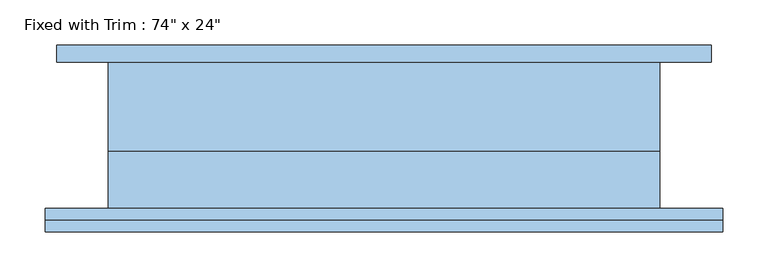
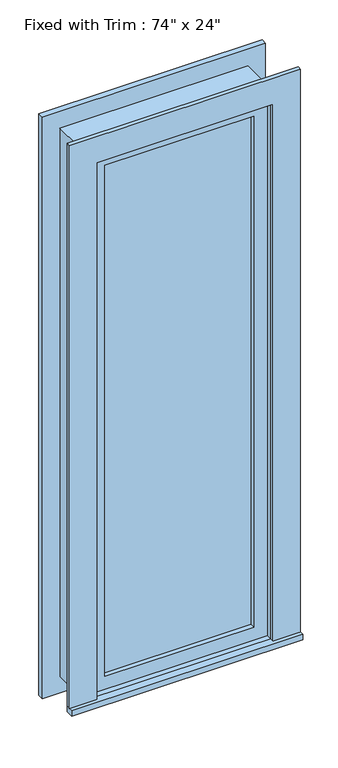
"""IFC4 building model written with IfcOpenShell, lengths in millimetres: window geometry."""

from ifc_helpers import new_model, si_unit, frame, origin, place, context, project, spatial, polyline, outline, extrude, source, transform, mapped, element, save


def window_368a6f6d(model_context):
    return source(origin(), model_context, "Body", "SweptSolid", [
        extrude(outline(polyline([(-412.75, -106.3625), (-412.75, -80.9625), (336.55, -80.9625), (336.55, -106.3625), (-412.75, -106.3625)])), frame((0.0, 0.0, 914.4), z_axis=(0.0, 0.0, 1.0), x_axis=(1.0, 0.0, 0.0)), (0.0, 0.0, 1.0), 19.05),
        extrude(outline(polyline([(2774.95, -323.85), (2774.95, 247.65), (933.45, 247.65), (933.45, 336.55), (2863.85, 336.55), (2863.85, -412.75), (933.45, -412.75), (933.45, -323.85), (2774.95, -323.85)])), frame((0.0, -93.6625, 0.0), z_axis=(0.0, 1.0, 0.0), x_axis=(0.0, 0.0, 1.0)), (0.0, 0.0, 1.0), 12.7),
        extrude(outline(polyline([(2851.15, 323.85), (2851.15, -400.05), (857.25, -400.05), (857.25, 323.85), (2851.15, 323.85)]), holes=[polyline([(2762.25, 234.95), (946.15, 234.95), (946.15, -311.15), (2762.25, -311.15), (2762.25, 234.95)])]), frame((0.0, 80.9625, 0.0), z_axis=(0.0, 1.0, 0.0), x_axis=(0.0, 0.0, 1.0)), (0.0, 0.0, 1.0), 19.05),
        extrude(outline(polyline([(203.2, -33.3375), (203.2, -46.0375), (-279.4, -46.0375), (-279.4, -33.3375), (203.2, -33.3375)])), frame((0.0, 0.0, 977.9), z_axis=(0.0, 0.0, 1.0), x_axis=(1.0, 0.0, 0.0)), (0.0, 0.0, 1.0), 1752.6),
        extrude(outline(polyline([(2774.95, -323.85), (933.45, -323.85), (933.45, 247.65), (2774.95, 247.65), (2774.95, -323.85)]), holes=[polyline([(2730.5, -279.4), (2730.5, 203.2), (977.9, 203.2), (977.9, -279.4), (2730.5, -279.4)])]), frame((0.0, -61.9125, 0.0), z_axis=(0.0, 1.0, 0.0), x_axis=(0.0, 0.0, 1.0)), (0.0, 0.0, 1.0), 44.45),
        extrude(outline(polyline([(2794.0, -342.9), (914.4, -342.9), (914.4, 266.7), (2794.0, 266.7), (2794.0, -342.9)]), holes=[polyline([(2762.25, -311.15), (2762.25, 234.95), (946.15, 234.95), (946.15, -311.15), (2762.25, -311.15)])]), frame((0.0, -17.4625, 0.0), z_axis=(0.0, 1.0, 0.0), x_axis=(0.0, 0.0, 1.0)), (0.0, 0.0, 1.0), 98.425),
        extrude(outline(polyline([(2794.0, 266.7), (2794.0, -342.9), (914.4, -342.9), (914.4, 266.7), (2794.0, 266.7)]), holes=[polyline([(2774.95, 247.65), (933.45, 247.65), (933.45, -323.85), (2774.95, -323.85), (2774.95, 247.65)])]), frame((0.0, -80.9625, 0.0), z_axis=(0.0, 1.0, 0.0), x_axis=(0.0, 0.0, 1.0)), (0.0, 0.0, 1.0), 63.5),
    ])


if __name__ == "__main__":
    model = new_model("IFC4")
    model_context = context("Model", 3, world=origin())
    ifc_project = project(units=[si_unit("LENGTHUNIT", "METRE", prefix="MILLI")], contexts=[model_context])
    site = spatial("IfcSite", under=ifc_project)
    building = spatial("IfcBuilding", under=site)
    placement = place(None, origin())
    window_shape = window_368a6f6d(model_context)
    element("IfcWindow", 1, ObjectType="Fixed with Trim : 74\" x 24\"", at=placement, inside=building, context=model_context, shape_type="MappedRepresentation", body=[
        mapped(window_shape, transform((0.0, 0.0, 0.0), x_axis=(1.0, 0.0, 0.0), y_axis=(0.0, 1.0, 0.0), z_axis=(0.0, 0.0, 1.0))),
    ])
    save(model, "model.ifc")

# Revit data of these elements
# Type "Fixed with Trim : 74\" x 24\""
#   Type Mark = "58"
#   COBie.Type.CreatedBy = "doug.wood@us.ibm.com"
#   COBie.Type.CreatedOn = "2016-04-14T02:07:26"
#   COBie.Type.Name = "Windows_Fixed with Trim_74\" x 24\"_58"
#   COBie.Type.Category = "23-30 20 17 11 : Fixed Windows"
#   COBie.Type.Description = "Fixed with Trim_74\" x 24\""
#   COBie.Type.Manufacturer = ""
#   COBie.Type.ModelNumber = ""
#   Construction Type Id = "GSP4R"
#   Assembly Code = "B2020100"
#   Analytic Construction = "1/8 in Pilkington single glazing"
#   COBie.Type.ReplacementCost = 0
#   Visual Light Transmittance = 0.9
#   Solar Heat Gain Coefficient = 0.78
#   Heat Transfer Coefficient (U) = 3.6886 W/(m²·K)
#   Height = 6' - 2"
#   Default Sill Height = 3' - 0"
#   Trim Projection - Ext. = 0' - 0 1/2"
#   Trim Projection - Int. = 0' - 0 3/4"
#   Trim Width - Exterior = 0' - 3 1/2"
#   Trim Width - Interior = 0' - 3 1/2"
#   Width = 2' - 0"
#   Window Inset = 0' - 0 3/4"
#   COBie.Type = no
#   Glass Pane Material = Glass
#   Sash Material = Sash - White
#   Trim Exterior Material = Trim - White
#   Trim Interior Material = Trim - White
#   Wall Closure = (empty or 0)
# Element 1 (IfcWindow, "Fixed with Trim : 74\" x 24\"")
#   Materials on its faces: "Sash - White", "Trim - White", "Glass"
# Materials
#   "Glass": class "Glass", colour RGB 0 128 192, transparency 0.75, Description = "Soda Lime Glass", Cost = 0
#   "Sash - White": class "Wood", colour RGB 255 255 255, transparency 0, Cost = 0
#   "Trim - White": class "Wood", colour RGB 255 255 255, transparency 0, Cost = 0
